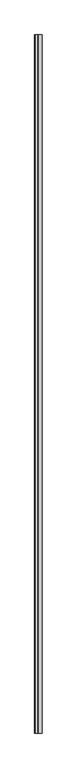
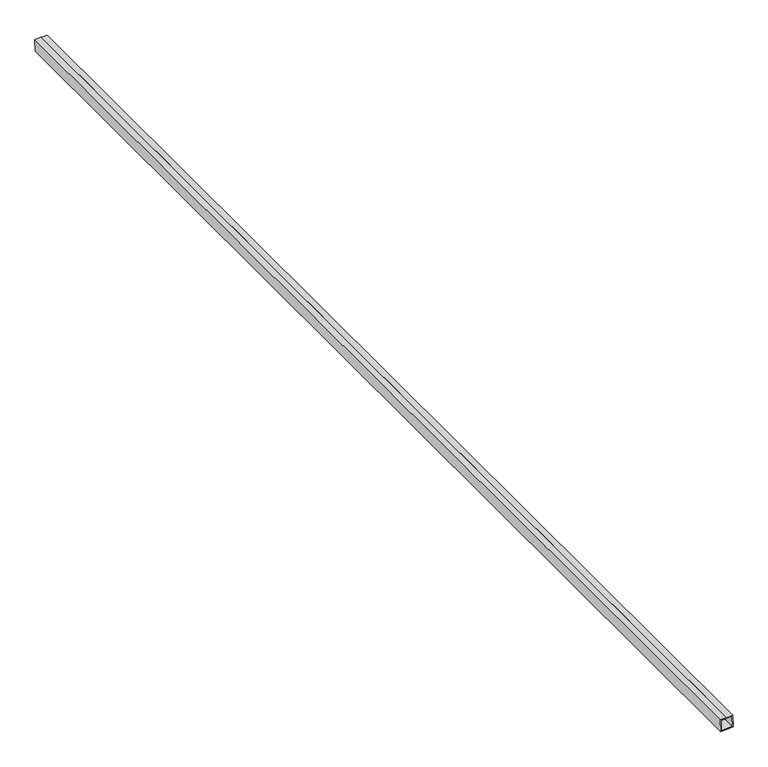
"""IFC4 building model written with IfcOpenShell, lengths in millimetres: proxy geometry, Inner panel:Inner panel:1:Inner panel:1 : Inner panel:Inner panel:300324:2:Inner panel:1:Inner panel:1 : Inner panel:Inner panel:300324:2 : Inner panel:Inner panel:1:Inner panel:1 : Inner panel:Inner panel:300324:300043:32 : Inner panel:Inner panel:1:Inner panel:1 : Inner panel:Inner panel:300324:2:Inner panel:1:Inner panel:1 : Inner panel:Inner panel:300324:2 : Inner panel:Inner panel:1:Inner panel:1 : Inner panel:Inner panel:300324:300043:308120."""

import ifcopenshell
import ifcopenshell.guid

model = None  # the IFC model being written
_history = None  # IfcOwnerHistory: only IFC2X3 demands one
_inside = {}  # id of a spatial element -> (the spatial element, [elements in it])
_under = {}  # id of a project, library or spatial element -> (it, [spatial elements below it])
_declared = {}  # id of a project -> (the project, [libraries it declares])
_typed = {}  # id of a type object -> (the type object, [elements of that type])
_made_of = {}  # id of a material, layer set ... -> (it, [elements and type objects made of it])


def new_model(schema):
    """Start an empty IFC model of exactly this schema.

    Asked for "IFC4X3", IfcOpenShell would pick the latest addendum, in which some entities
    have other attributes; the version numbers below select the first issue.
    IFC2X3 requires an IfcOwnerHistory on every rooted entity: one is made here for all.
    """
    global model, _history
    if schema == "IFC4X3":
        model = ifcopenshell.file(schema_version=(4, 3, 0, 0))
    else:
        model = ifcopenshell.file(schema=schema)
    _inside.clear()
    _under.clear()
    _declared.clear()
    _typed.clear()
    _made_of.clear()
    _history = None
    if model.schema == "IFC2X3":
        org = make("IfcOrganization", Name="unknown")
        user = make(
            "IfcPersonAndOrganization",
            ThePerson=make("IfcPerson", FamilyName="unknown"),
            TheOrganization=org,
        )
        app = make(
            "IfcApplication",
            ApplicationDeveloper=org,
            Version="unknown",
            ApplicationFullName="unknown",
            ApplicationIdentifier="unknown",
        )
        _history = make(
            "IfcOwnerHistory",
            OwningUser=user,
            OwningApplication=app,
            ChangeAction="ADDED",
            CreationDate=0,
        )
    return model


def make(cls, **values):
    """One entity of the class cls with the attributes given. An attribute that is None is left unset."""
    return model.create_entity(
        cls, **{name: value for name, value in values.items() if value is not None}
    )


def rooted(cls, **values):
    """An entity with a GlobalId (a new one), such as an element, a storey or a relation."""
    return make(cls, GlobalId=ifcopenshell.guid.new(), OwnerHistory=_history, **values)


def si_unit(unit_type, name, prefix=None):
    """IfcSIUnit, for example si_unit("LENGTHUNIT", "METRE", prefix="MILLI")."""
    return make("IfcSIUnit", UnitType=unit_type, Prefix=prefix, Name=name)


def assignment(units):
    """IfcUnitAssignment: the units of a project."""
    return None if units is None else make("IfcUnitAssignment", Units=units)


def point(xyz):
    """IfcCartesianPoint."""
    return None if xyz is None else make("IfcCartesianPoint", Coordinates=xyz)


def direction(xyz):
    """IfcDirection."""
    return None if xyz is None else make("IfcDirection", DirectionRatios=xyz)


def frame(location, z_axis=None, x_axis=None):
    """IfcAxis2Placement3D, a coordinate frame: its origin and axes. An axis left out is left unset."""
    return make(
        "IfcAxis2Placement3D",
        Location=point(location),
        Axis=direction(z_axis),
        RefDirection=direction(x_axis),
    )


def origin():
    """The frame at (0, 0, 0) with its axes left unset."""
    return frame((0.0, 0.0, 0.0))


def place(relative_to, where):
    """IfcLocalPlacement: puts the frame where relative to a parent placement (None: the world)."""
    return make(
        "IfcLocalPlacement", PlacementRelTo=relative_to, RelativePlacement=where
    )


def context(
    kind, dimensions, precision=None, world=None, true_north=None, identifier=None
):
    """IfcGeometricRepresentationContext, for example the 3D "Model" context."""
    return make(
        "IfcGeometricRepresentationContext",
        ContextIdentifier=identifier,
        ContextType=kind,
        CoordinateSpaceDimension=dimensions,
        Precision=precision,
        WorldCoordinateSystem=world,
        TrueNorth=true_north,
    )


def project(units=None, contexts=None):
    """IfcProject with its units and contexts."""
    return rooted(
        "IfcProject",
        Name="project",
        RepresentationContexts=contexts,
        UnitsInContext=assignment(units),
    )


def spatial(cls, under=None, at=None, **own):
    """A site, building, storey or space (cls), placed at a placement, below another one or the project."""
    s = rooted(cls, ObjectPlacement=at, **own)
    if under is not None:
        _under.setdefault(under.id(), (under, []))[1].append(s)
    return s


def polyline(points):
    """IfcPolyline through the points."""
    return make("IfcPolyline", Points=[point(p) for p in points])


def outline(outer, holes=None, kind="AREA"):
    """IfcArbitraryClosedProfileDef: a profile drawn as a closed curve; with holes, ...WithVoids."""
    if holes is None:
        return make("IfcArbitraryClosedProfileDef", ProfileType=kind, OuterCurve=outer)
    return make(
        "IfcArbitraryProfileDefWithVoids",
        ProfileType=kind,
        OuterCurve=outer,
        InnerCurves=holes,
    )


def extrude(swept, where, along, depth):
    """IfcExtrudedAreaSolid: the profile swept, set in the frame where, extruded along a direction by depth."""
    return make(
        "IfcExtrudedAreaSolid",
        SweptArea=swept,
        Position=where,
        ExtrudedDirection=direction(along),
        Depth=depth,
    )


def shape(context_of_items, identifier, shape_type, items):
    """IfcShapeRepresentation: the items that make up one representation, for example the "Body"."""
    return make(
        "IfcShapeRepresentation",
        ContextOfItems=context_of_items,
        RepresentationIdentifier=identifier,
        RepresentationType=shape_type,
        Items=items,
    )


def source(mapping_origin, context_of_items, identifier, shape_type, items):
    """IfcRepresentationMap: a shape defined once, which mapped items show again and again."""
    return make(
        "IfcRepresentationMap",
        MappingOrigin=mapping_origin,
        MappedRepresentation=shape(context_of_items, identifier, shape_type, items),
    )


def transform(
    local_origin,
    x_axis=None,
    y_axis=None,
    z_axis=None,
    scale=None,
    scale2=None,
    scale3=None,
    uniform=True,
):
    """IfcCartesianTransformationOperator3D, or its non-uniform kind. x_axis, y_axis, z_axis: its Axis1, 2, 3."""
    if uniform:
        return make(
            "IfcCartesianTransformationOperator3D",
            Axis1=direction(x_axis),
            Axis2=direction(y_axis),
            LocalOrigin=point(local_origin),
            Scale=scale,
            Axis3=direction(z_axis),
        )
    return make(
        "IfcCartesianTransformationOperator3DnonUniform",
        Axis1=direction(x_axis),
        Axis2=direction(y_axis),
        LocalOrigin=point(local_origin),
        Scale=scale,
        Axis3=direction(z_axis),
        Scale2=scale2,
        Scale3=scale3,
    )


def mapped(mapping_source, mapping_target):
    """IfcMappedItem: shows the shape of a source again, moved by a transform."""
    return make(
        "IfcMappedItem", MappingSource=mapping_source, MappingTarget=mapping_target
    )


def made_of(thing, what):
    """Note that an element or type object is made of a material, layer set ...; save() writes the relation."""
    if what is not None:
        _made_of.setdefault(what.id(), (what, []))[1].append(thing)
    return thing


def element(
    cls,
    number,
    at=None,
    inside=None,
    cuts=None,
    type_object=None,
    material=None,
    context=None,
    identifier="Body",
    shape_type=None,
    held_by="IfcProductDefinitionShape",
    body=None,
    shapes=None,
    **own,
):
    """One element of the class cls, such as IfcWall. Its Tag is "e" and its number.

    at: its placement. inside: the storey or other place that contains it. cuts: it is an
    opening in that element (IfcRelVoidsElement). A single representation is given by context,
    identifier, shape_type and body (its items); several are given by shapes. held_by: the class
    of the entity that holds the representations. save() writes the other relations.
    """
    e = rooted(cls, Tag="e%d" % number, ObjectPlacement=at, **own)
    if body is not None:
        shapes = [shape(context, identifier, shape_type, body)]
    if shapes is not None:
        e.Representation = make(held_by, Representations=shapes)
    if inside is not None:
        _inside.setdefault(inside.id(), (inside, []))[1].append(e)
    if cuts is not None:
        rooted(
            "IfcRelVoidsElement", RelatingBuildingElement=cuts, RelatedOpeningElement=e
        )
    if type_object is not None:
        _typed.setdefault(type_object.id(), (type_object, []))[1].append(e)
    return made_of(e, material)


def aggregate(whole, parts):
    """IfcRelAggregates: a whole, such as a stair, and the parts it consists of."""
    return rooted("IfcRelAggregates", RelatingObject=whole, RelatedObjects=parts)


def save(model, path):
    """Write the relations noted so far, then the file.

    IfcRelAggregates (storeys below a building ...), IfcRelContainedInSpatialStructure (elements
    in a storey), IfcRelDefinesByType, IfcRelAssociatesMaterial and IfcRelDeclares: one each for
    every whole, place, type object, material and project.
    """
    for whole, parts in _under.values():
        aggregate(whole, parts)
    for where, things in _inside.values():
        rooted(
            "IfcRelContainedInSpatialStructure",
            RelatedElements=things,
            RelatingStructure=where,
        )
    for kind, things in _typed.values():
        rooted("IfcRelDefinesByType", RelatedObjects=things, RelatingType=kind)
    for what, things in _made_of.values():
        rooted("IfcRelAssociatesMaterial", RelatedObjects=things, RelatingMaterial=what)
    for by, libraries in _declared.values():
        rooted("IfcRelDeclares", RelatingContext=by, RelatedDefinitions=libraries)
    model.write(path)


def generic_models_13fa0db4(model_context):
    return source(origin(), model_context, "Body", "SweptSolid", [
        extrude(outline(polyline([(3971.7309213, 560889.6434004), (3969.3517356, 560889.7425331), (3970.0126205, 560905.6037707), (3936.7040217, 560906.9916289), (3935.3161634, 560873.6830301), (3968.6247622, 560872.2951718), (3969.2856471, 560888.1564094), (3971.6648328, 560888.0572766), (3970.9048151, 560869.8168535), (3932.8378451, 560871.4029772), (3934.4239688, 560909.4699473), (3972.4909389, 560907.8838235), (3971.7309213, 560889.6434004)])), frame((0.0, -579334.066384, 0.0), z_axis=(0.0, 1.0, 0.0), x_axis=(0.0, 0.0, 1.0)), (0.0, 0.0, 1.0), 3657.6),
    ])


if __name__ == "__main__":
    model = new_model("IFC4")
    model_context = context("Model", 3, world=origin())
    ifc_project = project(units=[si_unit("LENGTHUNIT", "METRE", prefix="MILLI")], contexts=[model_context])
    site = spatial("IfcSite", under=ifc_project)
    building = spatial("IfcBuilding", under=site)
    placement = place(None, origin())
    generic_models_shape = generic_models_13fa0db4(model_context)
    element("IfcBuildingElementProxy", 1, Name="Inner panel:Inner panel:1:Inner panel:1 : Inner panel:Inner panel:300324:2:Inner panel:1:Inner panel:1 : Inner panel:Inner panel:300324:2 : Inner panel:Inner panel:1:Inner panel:1 : Inner panel:Inner panel:300324:300043:32 : Inner panel:Inner panel:1:Inner panel:1 : Inner panel:Inner panel:300324:2:Inner panel:1:Inner panel:1 : Inner panel:Inner panel:300324:2 : Inner panel:Inner panel:1:Inner panel:1 : Inner panel:Inner panel:300324:300043:308120", ObjectType="Inner panel:Inner panel:1:Inner panel:1 : Inner panel:Inner panel:300324:2:Inner panel:1:Inner panel:1 : Inner panel:Inner panel:300324:2 : Inner panel:Inner panel:1:Inner panel:1 : Inner panel:Inner panel:300324:300043:32 : Inner panel:Inner panel:1:Inner panel:1 : Inner panel:Inner panel:300324:2:Inner panel:1:Inner panel:1 : Inner panel:Inner panel:300324:2 : Inner panel:Inner panel:1:Inner panel:1 : Inner panel:Inner panel:300324:300043:308120", at=placement, inside=building, context=model_context, shape_type="MappedRepresentation", body=[
        mapped(generic_models_shape, transform((0.0, 0.0, 0.0), x_axis=(1.0, 0.0, 0.0), y_axis=(0.0, 1.0, 0.0), z_axis=(0.0, 0.0, 1.0))),
    ])
    save(model, "model.ifc")

# Revit data of these elements
# Type "Inner panel:Inner panel:1:Inner panel:1 : Inner panel:Inner panel:300324:2:Inner panel:1:Inner panel:1 : Inner panel:Inner panel:300324:2 : Inner panel:Inner panel:1:Inner panel:1 : Inner panel:Inner panel:300324:300043:32 : Inner panel:Inner panel:1:Inner panel:1 : Inner panel:Inner panel:300324:2:Inner panel:1:Inner panel:1 : Inner panel:Inner panel:300324:2 : Inner panel:Inner panel:1:Inner panel:1 : Inner panel:Inner panel:300324:300043:308120"
#   NameOverride = "Inner panel:Inner panel:1:Inner panel:1 : Inner panel:Inner panel:300324:2:Inner panel:1:Inner panel:1 : Inner panel:Inner panel:300324:2 : Inner panel:Inner panel:1:Inner panel:1 : Inner panel:Inner panel:300324:300043:308120"
#   ObjectTypeOverride = "Inner panel:1:Inner panel:1 : Inner panel:Inner panel:300324:2 : Inner panel:Inner panel:1:Inner panel:1 : Inner panel:Inner panel:300324:300043"
#   Reference = "Inner panel"
#   Tag = "308120"
# Element 1 (IfcBuildingElementProxy, "Inner panel:Inner panel:1:Inner panel:1 : Inner panel:Inner panel:300324:2:Inner panel:1:Inner panel:1 : Inner panel:Inner panel:300324:2 : Inner panel:Inner panel:1:Inner panel:1 : Inner panel:Inner panel:300324:300043:32 : Inner panel:Inner panel:1:Inner panel:1 : Inner panel:Inner panel:300324:2:Inner panel:1:Inner panel:1 : Inner panel:Inner panel:300324:2 : Inner panel:Inner panel:1:Inner panel:1 : Inner panel:Inner panel:300324:300043:308120")
#   Materials on its faces: "1 1/2\" X 1 1/2\" SPLIT-SEAM SQUARE TUBING (~24\" CANTILEVER FROM C.L. OF GLULAM)"
# Materials
#   "1 1/2\" X 1 1/2\" SPLIT-SEAM SQUARE TUBING (~24\" CANTILEVER FROM C.L. OF GLULAM)": class "Unassigned", colour RGB 202 201 200, transparency 0, Cost = 0
